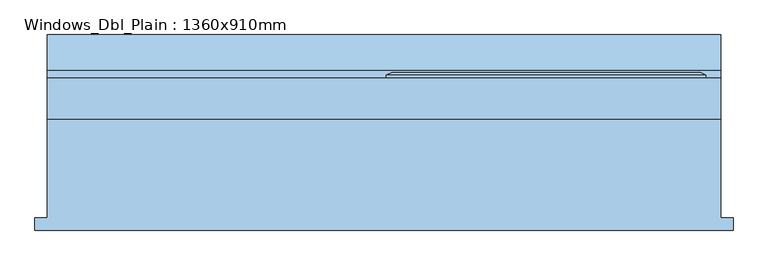
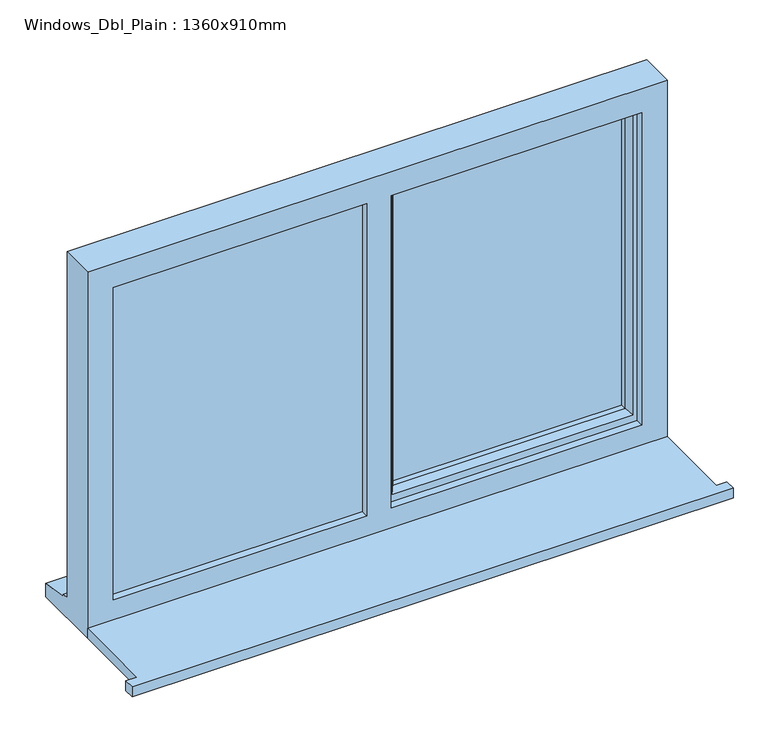
"""IFC4 building model written with IfcOpenShell, lengths in millimetres: window geometry, Windows_Dbl_Plain : 1360x910mm."""

from ifc_helpers import new_model, si_unit, frame, origin, place, context, project, spatial, polyline, outline, extrude, faceted_brep, source, transform, mapped, element, save


def windows_dbl_plain_1360x910mm_a67c5c4d(model_context):
    return source(origin(), model_context, "Body", "SolidModel", [
        extrude(outline(polyline([(-990.0, -182.7934322), (-990.0, -157.7934322), (-965.0, -157.7934322), (-965.0, 41.7065678), (395.0, 41.7065678), (395.0, -157.7934322), (420.0, -157.7934322), (420.0, -182.7934322), (-990.0, -182.7934322)])), frame((0.0, 0.0, 1200.0), z_axis=(0.0, 0.0, 1.0), x_axis=(1.0, 0.0, 0.0)), (0.0, 0.0, 1.0), 25.0),
        extrude(outline(polyline([(325.0, 88.7065678), (-240.0, 88.7065678), (-240.0, 112.7065678), (325.0, 112.7065678), (325.0, 88.7065678)])), frame((0.0, 0.0, 1293.0), z_axis=(0.0, 0.0, 1.0), x_axis=(1.0, 0.0, 0.0)), (0.0, 0.0, 1.0), 747.0),
        extrude(outline(polyline([(-925.0, 83.7065678), (-300.0, 83.7065678), (-300.0, 59.7065678), (-925.0, 59.7065678), (-925.0, 83.7065678)])), frame((0.0, 0.0, 1263.0), z_axis=(0.0, 0.0, 1.0), x_axis=(1.0, 0.0, 0.0)), (0.0, 0.0, 1.0), 807.0),
        faceted_brep([(395.0, 41.7065678, 2110.0), (-965.0, 41.7065678, 2110.0), (-965.0, 41.7065678, 1200.0), (395.0, 41.7065678, 1200.0), (335.0, 41.7065678, 2050.0), (335.0, 41.7065678, 1275.0), (-252.0, 41.7065678, 1275.0), (-252.0, 41.7065678, 2050.0), (-310.0, 41.7065678, 2050.0), (-310.0, 41.7065678, 1275.0), (-905.0, 41.7065678, 1275.0), (-905.0, 41.7065678, 2050.0), (-965.0, 124.7065678, 2110.0), (-965.0, 124.7065678, 1251.0), (-965.0, 139.7065678, 1249.68767), (-965.0, 139.7065678, 1244.7449676), (-965.0, 212.2065678, 1233.8088847), (-965.0, 212.2065678, 1200.0), (395.0, 124.7065678, 2110.0), (395.0, 124.7065678, 1251.0), (-925.0, 124.7065678, 2070.0), (-925.0, 124.7065678, 1263.0), (-310.0, 124.7065678, 1263.0), (-310.0, 124.7065678, 2070.0), (-270.0, 124.7065678, 2070.0), (-270.0, 124.7065678, 1263.0), (355.0, 124.7065678, 1263.0), (355.0, 124.7065678, 2070.0), (-925.0, 59.7065678, 2070.0), (-925.0, 59.7065678, 1263.0), (-300.0, 59.7065678, 2070.0), (-300.0, 59.7065678, 1263.0), (-310.0, 59.7065678, 2050.0), (-905.0, 59.7065678, 2050.0), (-905.0, 59.7065678, 1275.0), (-310.0, 59.7065678, 1275.0), (-270.0, 59.7065678, 2070.0), (355.0, 59.7065678, 2070.0), (355.0, 59.7065678, 1263.0), (-270.0, 59.7065678, 1263.0), (335.0, 59.7065678, 2050.0), (-252.0, 59.7065678, 2050.0), (-252.0, 59.7065678, 1275.0), (335.0, 59.7065678, 1275.0), (-310.0, 83.7065678, 2070.0), (-300.0, 83.7065678, 2070.0), (395.0, 212.2065678, 1200.0), (395.0, 212.2065678, 1233.8088847), (395.0, 139.7065678, 1244.7449676), (395.0, 139.7065678, 1249.68767), (-300.0, 83.7065678, 1263.0), (-310.0, 83.7065678, 1263.0)], [[[0, 1, 2, 3], [4, 5, 6, 7], [8, 9, 10, 11]], [[2, 1, 12, 13, 14, 15, 16, 17]], [[13, 12, 18, 19], [20, 21, 22, 23], [24, 25, 26, 27]], [[21, 20, 28, 29]], [[28, 30, 31, 29], [32, 33, 34, 35]], [[36, 37, 38, 39], [40, 41, 42, 43]], [[33, 11, 10, 34]], [[1, 0, 18, 12]], [[28, 20, 23, 44, 45, 30]], [[27, 37, 36, 24]], [[11, 33, 32, 8]], [[40, 4, 7, 41]], [[19, 18, 0, 3, 46, 47, 48, 49]], [[27, 26, 38, 37]], [[4, 40, 43, 5]], [[45, 50, 31, 30]], [[50, 45, 44, 51]], [[51, 44, 23, 22]], [[25, 24, 36, 39]], [[41, 7, 6, 42]], [[8, 32, 35, 9]], [[46, 3, 2, 17]], [[47, 46, 17, 16]], [[48, 47, 16, 15]], [[49, 48, 15, 14]], [[19, 49, 14, 13]], [[22, 21, 29, 31, 50, 51]], [[26, 25, 39, 38]], [[6, 5, 43, 42]], [[35, 34, 10, 9]]]),
        extrude(outline(polyline([(2050.0, -310.0), (2070.0, -310.0), (2070.0, -925.0), (1263.0, -925.0), (1263.0, -310.0), (1283.0, -310.0), (1283.0, -905.0), (2050.0, -905.0), (2050.0, -310.0)])), frame((0.0, 83.7065678, 0.0), z_axis=(0.0, 1.0, 0.0), x_axis=(0.0, 0.0, 1.0)), (0.0, 0.0, 1.0), 41.0),
        faceted_brep([(-280.0, 124.7065678, 2080.0), (-280.0, 130.4800705, 2080.0), (-280.0, 130.4800705, 1253.0), (-280.0, 124.7065678, 1253.0), (-270.0, 59.7065678, 2070.0), (-270.0, 124.7065678, 2070.0), (-270.0, 124.7065678, 1263.0), (-270.0, 59.7065678, 1263.0), (-230.0, 74.1994677, 2030.0), (-240.1480377, 59.7065678, 2040.1480377), (-240.1480377, 59.7065678, 1292.8519623), (-230.0, 74.1994677, 1303.0), (-230.0, 88.7065678, 2030.0), (-230.0, 88.7065678, 1303.0), (-240.0, 112.7065678, 2040.0), (-240.0, 88.7065678, 2040.0), (-240.0, 88.7065678, 1293.0), (-240.0, 112.7065678, 1293.0), (-230.0, 130.4800705, 2030.0), (-230.0, 112.7065678, 2030.0), (-230.0, 112.7065678, 1303.0), (-230.0, 130.4800705, 1303.0), (-247.4457548, 136.2535732, 2047.4457548), (-247.4457548, 136.2535732, 1285.5542452), (-269.2153903, 136.2535732, 2069.2153903), (-269.2153903, 136.2535732, 1263.7846097), (365.0, 130.4800705, 1253.0), (365.0, 124.7065678, 1253.0), (355.0, 124.7065678, 1263.0), (355.0, 59.7065678, 1263.0), (325.1480377, 59.7065678, 1292.8519623), (315.0, 74.1994677, 1303.0), (315.0, 88.7065678, 1303.0), (325.0, 88.7065678, 1293.0), (325.0, 112.7065678, 1293.0), (315.0, 112.7065678, 1303.0), (315.0, 130.4800705, 1303.0), (332.4457548, 136.2535732, 1285.5542452), (354.2153903, 136.2535732, 1263.7846097), (365.0, 130.4800705, 2080.0), (365.0, 124.7065678, 2080.0), (355.0, 124.7065678, 2070.0), (355.0, 59.7065678, 2070.0), (325.1480377, 59.7065678, 2040.1480377), (315.0, 74.1994677, 2030.0), (315.0, 88.7065678, 2030.0), (325.0, 88.7065678, 2040.0), (325.0, 112.7065678, 2040.0), (315.0, 112.7065678, 2030.0), (315.0, 130.4800705, 2030.0), (332.4457548, 136.2535732, 2047.4457548), (354.2153903, 136.2535732, 2069.2153903)], [[[0, 1, 2, 3]], [[4, 5, 6, 7]], [[8, 9, 10, 11]], [[12, 8, 11, 13]], [[14, 15, 16, 17]], [[18, 19, 20, 21]], [[22, 18, 21, 23]], [[1, 24, 25, 2]], [[3, 2, 26, 27]], [[7, 6, 28, 29]], [[11, 10, 30, 31]], [[13, 11, 31, 32]], [[17, 16, 33, 34]], [[21, 20, 35, 36]], [[23, 21, 36, 37]], [[2, 25, 38, 26]], [[27, 26, 39, 40]], [[29, 28, 41, 42]], [[31, 30, 43, 44]], [[32, 31, 44, 45]], [[34, 33, 46, 47]], [[36, 35, 48, 49]], [[37, 36, 49, 50]], [[26, 38, 51, 39]], [[40, 39, 1, 0]], [[3, 27, 40, 0], [5, 41, 28, 6]], [[42, 41, 5, 4]], [[7, 29, 42, 4], [9, 43, 30, 10]], [[44, 43, 9, 8]], [[45, 44, 8, 12]], [[15, 46, 33, 16], [13, 32, 45, 12]], [[47, 46, 15, 14]], [[17, 34, 47, 14], [19, 48, 35, 20]], [[49, 48, 19, 18]], [[50, 49, 18, 22]], [[24, 51, 38, 25], [23, 37, 50, 22]], [[39, 51, 24, 1]]]),
    ])


if __name__ == "__main__":
    model = new_model("IFC4")
    model_context = context("Model", 3, world=origin())
    ifc_project = project(units=[si_unit("LENGTHUNIT", "METRE", prefix="MILLI")], contexts=[model_context])
    site = spatial("IfcSite", under=ifc_project)
    building = spatial("IfcBuilding", under=site)
    placement = place(None, origin())
    windows_dbl_plain_1360x910mm_shape = windows_dbl_plain_1360x910mm_a67c5c4d(model_context)
    element("IfcWindow", 1, ObjectType="Windows_Dbl_Plain : 1360x910mm", at=placement, inside=building, context=model_context, shape_type="MappedRepresentation", body=[
        mapped(windows_dbl_plain_1360x910mm_shape, transform((0.0, 0.0, 0.0), x_axis=(1.0, 0.0, 0.0), y_axis=(0.0, 1.0, 0.0), z_axis=(0.0, 0.0, 1.0))),
    ])
    save(model, "model.ifc")

# Revit data of these elements
# Type "Windows_Dbl_Plain : 1360x910mm"
#   Type Mark = "82"
#   Operation = "DoublePanelVertical"
#   Construction Type Id = "GSP4R"
#   Manufacturer = "Revit"
#   Keynote = "L10"
#   Analytic Construction = "1/8 in Pilkington single glazing"
#   Wrap Layers (Ext) from Ext = 102.5 mm
#   Wrap Layers (Int) from Ext = 177.5 mm
#   Window Board Projection = 25 mm
#   Window Board Extension = 25 mm
#   Visual Light Transmittance = 0.9
#   Solar Heat Gain Coefficient = 0.78
#   Rough Width = 1360 mm
#   Rough Height = 910 mm
#   Height = 910 mm
#   Width = 1360 mm
#   Heat Transfer Coefficient (U) = 3.6886 W/(m²·K)
#   Glazing Thickness = 24 mm
#   FrameOffset - External = 50 mm
#   Frame Depth = 65 mm
#   Default Head Height = 2110 mm
#   Cill Depth = 87.5 mm
#   Cavity Closer Width = 50 mm
#   Cavity Closer Offset from Ext = 102.5 mm
#   Cavity Closer Depth = 85 mm
#   Vis - Cavity Closers = yes
#   Define Thermal Properties by = 1
#   Material Trim = Window Frame
#   Material Glass = Glass
#   Material Frame = Window Frame
#   Wall Closure = (empty or 0)
# Element 1 (IfcWindow, "Windows_Dbl_Plain : 1360x910mm")
#   Materials on its faces: "Window Frame", "Glass"
# Materials
#   "Window Frame": class "Miscellaneous", colour RGB 249 249 249, transparency 0, Keynote = "L10"
#   "Glass": class "Glass", colour RGB 0 128 192, transparency 0.9, Description = "Soda Lime Glass", Cost = 0
